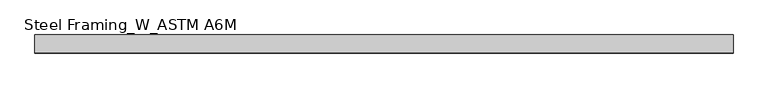
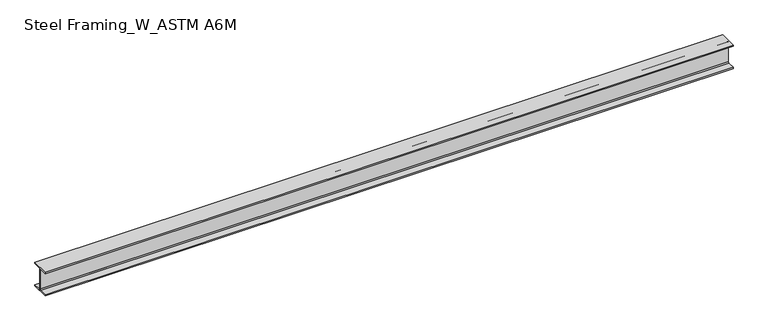
"""IFC4 building model written with IfcOpenShell, lengths in millimetres: beam geometry, Steel Framing_W_ASTM A6M : H_SB_AR_S02_W360x91_B3."""

from ifc_helpers import new_model, si_unit, point, frame, frame_2d, origin, place, context, project, spatial, polyline, circle_curve, trimmed, segment, composite_curve, outline, extrude, source, transform, mapped, element, save


def steel_framing_w_astm_a6m_c8525865(model_context):
    return source(origin(), model_context, "Body", "SweptSolid", [
        extrude(outline(composite_curve([segment(polyline([(127.0, -160.1), (127.0, -176.5), (-127.0, -176.5), (-127.0, -160.1), (-19.865, -160.1)]), True, "CONTINUOUS"), segment(trimmed(circle_curve(frame_2d((-19.865, -145.0)), 15.1), [point((-19.865, -160.1))], [point((-4.765, -145.0))], True, "CARTESIAN"), True, "CONTINUOUS"), segment(polyline([(-4.765, -145.0), (-4.765, 145.0)]), True, "CONTINUOUS"), segment(trimmed(circle_curve(frame_2d((-19.865, 145.0)), 15.1), [point((-4.765, 145.0))], [point((-19.865, 160.1))], True, "CARTESIAN"), True, "CONTINUOUS"), segment(polyline([(-19.865, 160.1), (-127.0, 160.1), (-127.0, 176.5), (127.0, 176.5), (127.0, 160.1), (19.865, 160.1)]), True, "CONTINUOUS"), segment(trimmed(circle_curve(frame_2d((19.865, 145.0)), 15.1), [point((19.865, 160.1))], [point((4.765, 145.0))], True, "CARTESIAN"), True, "CONTINUOUS"), segment(polyline([(4.765, 145.0), (4.765, -145.0)]), True, "CONTINUOUS"), segment(trimmed(circle_curve(frame_2d((19.865, -145.0)), 15.1), [point((4.765, -145.0))], [point((19.865, -160.1))], True, "CARTESIAN"), True, "CONTINUOUS"), segment(polyline([(19.865, -160.1), (127.0, -160.1)]), True, "CONTINUOUS")], self_intersect=False)), frame((-4901.8, 0.0, 0.0), z_axis=(1.0, 0.0, 0.0), x_axis=(0.0, 1.0, 0.0)), (0.0, 0.0, 1.0), 9803.6),
    ])


if __name__ == "__main__":
    model = new_model("IFC4")
    model_context = context("Model", 3, world=origin())
    ifc_project = project(units=[si_unit("LENGTHUNIT", "METRE", prefix="MILLI")], contexts=[model_context])
    site = spatial("IfcSite", under=ifc_project)
    building = spatial("IfcBuilding", under=site)
    placement = place(None, origin())
    steel_framing_w_astm_a6m_shape = steel_framing_w_astm_a6m_c8525865(model_context)
    element("IfcBeam", 1, ObjectType="Steel Framing_W_ASTM A6M : H_SB_AR_S02_W360x91_B3", at=placement, inside=building, context=model_context, shape_type="MappedRepresentation", body=[
        mapped(steel_framing_w_astm_a6m_shape, transform((0.0, 0.0, 0.0), x_axis=(1.0, 0.0, 0.0), y_axis=(0.0, 1.0, 0.0), z_axis=(0.0, 0.0, 1.0))),
    ])
    save(model, "model.ifc")

# Revit data of these elements
# Type "Steel Framing_W_ASTM A6M : H_SB_AR_S02_W360x91_B3"
#   Type Mark = "B3"
#   Section Name Key = "W14x61"
#   Width = 25.4 cm
#   Web Thickness = 0.953 cm
#   Web Fillet = 1.51 cm
#   Warping Constant = 1260000.0 cm⁶
#   Torsional Moment of Inertia = 91.20 cm⁴
#   Section Area = 115.0 cm²
#   Plastic Modulus weak axis = 537.0 cm³
#   Plastic Modulus strong axis = 1670.0 cm³
#   Perimeter = 1.68 m²/m
#   Nominal Weight = 91.00 kgf/m
#   Moment of Inertia weak axis = 4450.00 cm⁴
#   Moment of Inertia strong axis = 26600.00 cm⁴
#   Height = 35.3 cm
#   Flange Thickness = 1.64 cm
#   Elastic Modulus weak axis = 352.0 cm³
#   Elastic Modulus strong axis = 1510.0 cm³
#   Centroid Vertical = 17.65 cm
#   Centroid Horizontal = 12.7 cm
#   Length [instance default] = 1500 mm
#   Structural Material [instance default] = Steel, 45-345
#   Bolt Spacing = 0
#   Assembly Code = ""
# Element 1 (IfcBeam, "Steel Framing_W_ASTM A6M : H_SB_AR_S02_W360x91_B3")
#   Materials on its faces: "Steel, 45-345"
# Materials
#   "Steel, 45-345": class "Metal", colour RGB 189 187 185, transparency 0, Description = "Steel 345 MPa", Cost = 0
